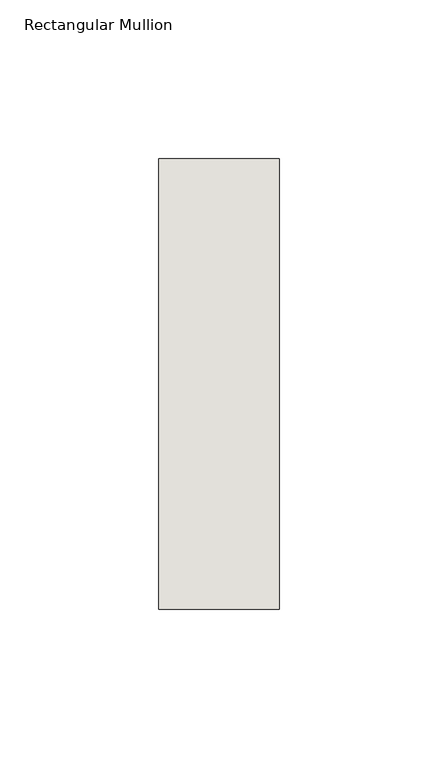
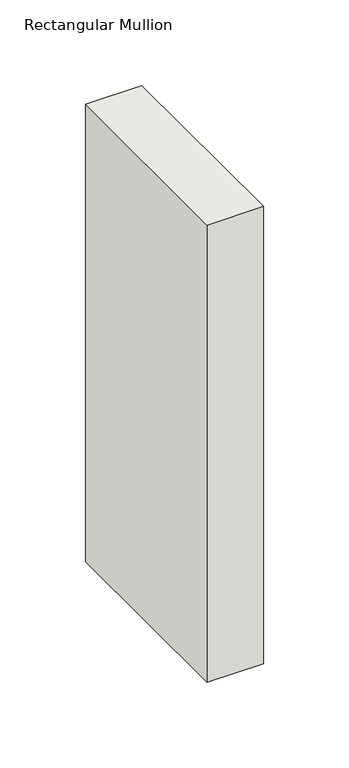
"""IFC4 building model written with IfcOpenShell, lengths in millimetres: wall geometry, Rectangular Mullion : NLRS_21_CWM_hsb-regel 38x142_gen_rsf."""

from ifc_helpers import new_model, si_unit, frame, origin, place, context, project, spatial, polyline, outline, extrude, source, transform, mapped, element, save


def rectangular_mullion_610e01e3(model_context):
    return source(origin(), model_context, "Body", "SweptSolid", [
        extrude(outline(polyline([(0.0, -71.0), (-38.0, -71.0), (-38.0, 71.0), (0.0, 71.0), (0.0, -71.0)])), frame((0.0, 0.0, -326.0000003), z_axis=(0.0, 0.0, 1.0), x_axis=(1.0, 0.0, 0.0)), (0.0, 0.0, 1.0), 326.0000003),
    ])


if __name__ == "__main__":
    model = new_model("IFC4")
    model_context = context("Model", 3, world=origin())
    ifc_project = project(units=[si_unit("LENGTHUNIT", "METRE", prefix="MILLI")], contexts=[model_context])
    site = spatial("IfcSite", under=ifc_project)
    building = spatial("IfcBuilding", under=site)
    placement = place(None, origin())
    rectangular_mullion_shape = rectangular_mullion_610e01e3(model_context)
    element("IfcWall", 1, ObjectType="Rectangular Mullion : NLRS_21_CWM_hsb-regel 38x142_gen_rsf", at=placement, inside=building, context=model_context, shape_type="MappedRepresentation", body=[
        mapped(rectangular_mullion_shape, transform((0.0, 0.0, 0.0), x_axis=(1.0, 0.0, 0.0), y_axis=(0.0, 1.0, 0.0), z_axis=(0.0, 0.0, 1.0))),
    ])
    save(model, "model.ifc")

# Revit data of these elements
# Type "Rectangular Mullion : NLRS_21_CWM_hsb-regel 38x142_gen_rsf"
#   Type IfcGUID = "07M7mRoiH1CR8m_RSKIwpF"
#   Assembly Code = "21.10"
#   IfcExportAs = "IfcWall"
#   built-in parameter 1007322 = 0.465879 (stored number, unit not read)
#   built-in parameter 1007321 = 0.062336 (stored number, unit not read)
#   built-in parameter 1007320 = 0.062336 (stored number, unit not read)
# Element 1 (IfcWall, "Rectangular Mullion : NLRS_21_CWM_hsb-regel 38x142_gen_rsf")
#   Materials on its faces: "NLRS_i2_hout naaldhout vuren_gen_rsf"
# Materials
#   "NLRS_i2_hout naaldhout vuren_gen_rsf": class "I - Hout", colour RGB 234 199 147, transparency 0, Keynote = "i2", Manufacturer = "Revit Standards Foundation", URL = "www.revitstandards.org", Description = "hout vuren", Cost = 0
